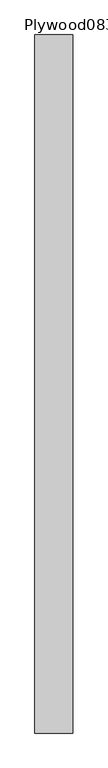
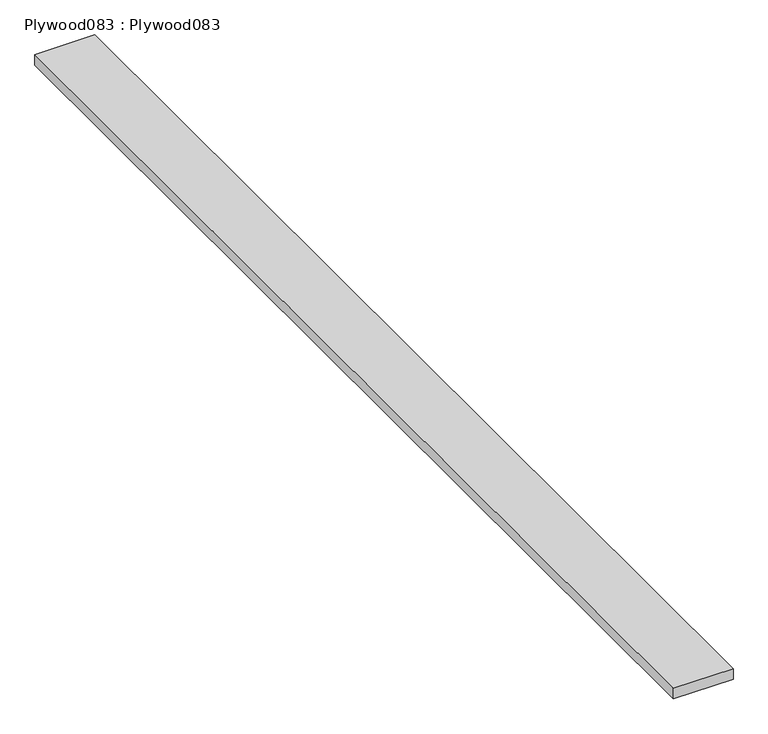
"""IFC4 building model written with IfcOpenShell, lengths in millimetres: proxy geometry, Plywood083 : Plywood083."""

from ifc_helpers import new_model, si_unit, frame, origin, place, context, project, spatial, polyline, outline, extrude, source, transform, mapped, element, save


def plywood083_plywood083_54aaa039(model_context):
    return source(origin(), model_context, "Body", "SweptSolid", [
        extrude(outline(polyline([(-950.3815411, -1052.8906574), (-1058.630127, -1052.8906574), (-1058.630127, 947.1093426), (-950.3815411, 947.1093426), (-950.3815411, -1052.8906574)])), frame((0.0, 0.0, 40315.896), z_axis=(0.0, 0.0, 1.0), x_axis=(1.0, 0.0, 0.0)), (0.0, 0.0, 1.0), 19.9461875),
    ])


if __name__ == "__main__":
    model = new_model("IFC4")
    model_context = context("Model", 3, world=origin())
    ifc_project = project(units=[si_unit("LENGTHUNIT", "METRE", prefix="MILLI")], contexts=[model_context])
    site = spatial("IfcSite", under=ifc_project)
    building = spatial("IfcBuilding", under=site)
    placement = place(None, origin())
    plywood083_plywood083_shape = plywood083_plywood083_54aaa039(model_context)
    element("IfcBuildingElementProxy", 1, Name="Plywood083 : Plywood083", ObjectType="Plywood083 : Plywood083", at=placement, inside=building, context=model_context, shape_type="MappedRepresentation", body=[
        mapped(plywood083_plywood083_shape, transform((0.0, 0.0, 0.0), x_axis=(1.0, 0.0, 0.0), y_axis=(0.0, 1.0, 0.0), z_axis=(0.0, 0.0, 1.0))),
    ])
    save(model, "model.ifc")

# Revit data of these elements
# Type "Plywood083 : Plywood083"
#   NameOverride = "Plywood083"
# Element 1 (IfcBuildingElementProxy, "Plywood083 : Plywood083")
#   Materials on its faces: "5/8\" GYPSUM BOARD"
# Materials
#   "5/8\" GYPSUM BOARD": class "Unassigned", colour RGB 255 255 255, transparency 0, Cost = 0
